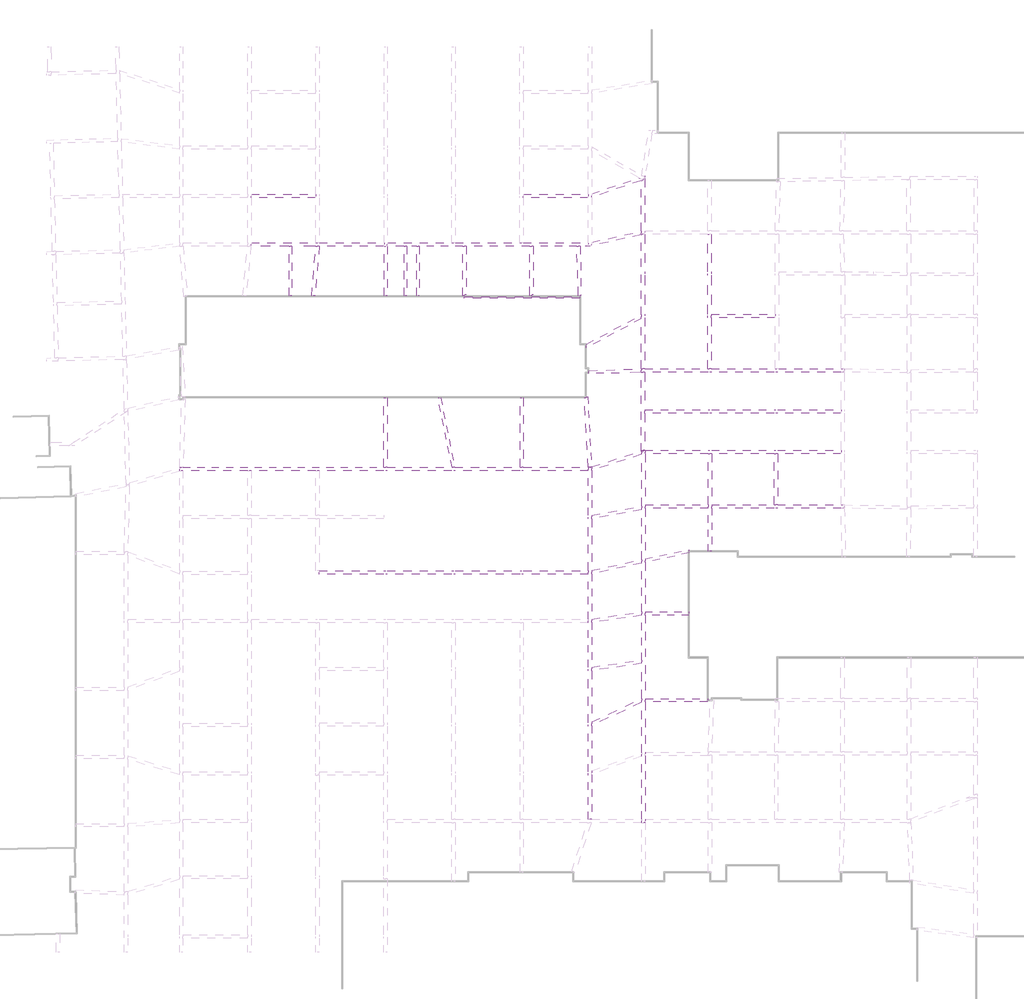
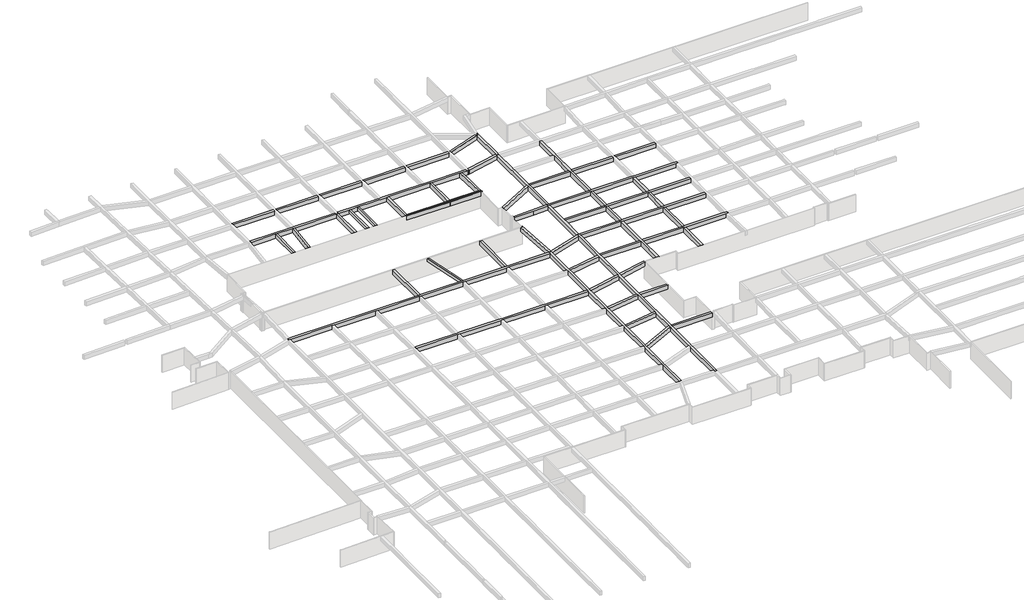
# One storey, part 12 of 20: 47 beams.
"""IFC4 building model written with IfcOpenShell, lengths in millimetres."""

import ifcopenshell
import ifcopenshell.guid

model = None  # the IFC model being written
_history = None  # IfcOwnerHistory: only IFC2X3 demands one
_inside = {}  # id of a spatial element -> (the spatial element, [elements in it])
_under = {}  # id of a project, library or spatial element -> (it, [spatial elements below it])
_declared = {}  # id of a project -> (the project, [libraries it declares])
_typed = {}  # id of a type object -> (the type object, [elements of that type])
_made_of = {}  # id of a material, layer set ... -> (it, [elements and type objects made of it])


def new_model(schema):
    """Start an empty IFC model of exactly this schema.

    Asked for "IFC4X3", IfcOpenShell would pick the latest addendum, in which some entities
    have other attributes; the version numbers below select the first issue.
    IFC2X3 requires an IfcOwnerHistory on every rooted entity: one is made here for all.
    """
    global model, _history
    if schema == "IFC4X3":
        model = ifcopenshell.file(schema_version=(4, 3, 0, 0))
    else:
        model = ifcopenshell.file(schema=schema)
    _inside.clear()
    _under.clear()
    _declared.clear()
    _typed.clear()
    _made_of.clear()
    _history = None
    if model.schema == "IFC2X3":
        org = make("IfcOrganization", Name="unknown")
        user = make(
            "IfcPersonAndOrganization",
            ThePerson=make("IfcPerson", FamilyName="unknown"),
            TheOrganization=org,
        )
        app = make(
            "IfcApplication",
            ApplicationDeveloper=org,
            Version="unknown",
            ApplicationFullName="unknown",
            ApplicationIdentifier="unknown",
        )
        _history = make(
            "IfcOwnerHistory",
            OwningUser=user,
            OwningApplication=app,
            ChangeAction="ADDED",
            CreationDate=0,
        )
    return model


def make(cls, **values):
    """One entity of the class cls with the attributes given. An attribute that is None is left unset."""
    return model.create_entity(
        cls, **{name: value for name, value in values.items() if value is not None}
    )


def rooted(cls, **values):
    """An entity with a GlobalId (a new one), such as an element, a storey or a relation."""
    return make(cls, GlobalId=ifcopenshell.guid.new(), OwnerHistory=_history, **values)


def si_unit(unit_type, name, prefix=None):
    """IfcSIUnit, for example si_unit("LENGTHUNIT", "METRE", prefix="MILLI")."""
    return make("IfcSIUnit", UnitType=unit_type, Prefix=prefix, Name=name)


def assignment(units):
    """IfcUnitAssignment: the units of a project."""
    return None if units is None else make("IfcUnitAssignment", Units=units)


def point(xyz):
    """IfcCartesianPoint."""
    return None if xyz is None else make("IfcCartesianPoint", Coordinates=xyz)


def direction(xyz):
    """IfcDirection."""
    return None if xyz is None else make("IfcDirection", DirectionRatios=xyz)


def frame(location, z_axis=None, x_axis=None):
    """IfcAxis2Placement3D, a coordinate frame: its origin and axes. An axis left out is left unset."""
    return make(
        "IfcAxis2Placement3D",
        Location=point(location),
        Axis=direction(z_axis),
        RefDirection=direction(x_axis),
    )


def origin():
    """The frame at (0, 0, 0) with its axes left unset."""
    return frame((0.0, 0.0, 0.0))


def place(relative_to, where):
    """IfcLocalPlacement: puts the frame where relative to a parent placement (None: the world)."""
    return make(
        "IfcLocalPlacement", PlacementRelTo=relative_to, RelativePlacement=where
    )


def context(
    kind, dimensions, precision=None, world=None, true_north=None, identifier=None
):
    """IfcGeometricRepresentationContext, for example the 3D "Model" context."""
    return make(
        "IfcGeometricRepresentationContext",
        ContextIdentifier=identifier,
        ContextType=kind,
        CoordinateSpaceDimension=dimensions,
        Precision=precision,
        WorldCoordinateSystem=world,
        TrueNorth=true_north,
    )


def project(units=None, contexts=None):
    """IfcProject with its units and contexts."""
    return rooted(
        "IfcProject",
        Name="project",
        RepresentationContexts=contexts,
        UnitsInContext=assignment(units),
    )


def spatial(cls, under=None, at=None, **own):
    """A site, building, storey or space (cls), placed at a placement, below another one or the project."""
    s = rooted(cls, ObjectPlacement=at, **own)
    if under is not None:
        _under.setdefault(under.id(), (under, []))[1].append(s)
    return s


def polyline(points):
    """IfcPolyline through the points."""
    return make("IfcPolyline", Points=[point(p) for p in points])


def outline(outer, holes=None, kind="AREA"):
    """IfcArbitraryClosedProfileDef: a profile drawn as a closed curve; with holes, ...WithVoids."""
    if holes is None:
        return make("IfcArbitraryClosedProfileDef", ProfileType=kind, OuterCurve=outer)
    return make(
        "IfcArbitraryProfileDefWithVoids",
        ProfileType=kind,
        OuterCurve=outer,
        InnerCurves=holes,
    )


def extrude(swept, where, along, depth):
    """IfcExtrudedAreaSolid: the profile swept, set in the frame where, extruded along a direction by depth."""
    return make(
        "IfcExtrudedAreaSolid",
        SweptArea=swept,
        Position=where,
        ExtrudedDirection=direction(along),
        Depth=depth,
    )


def faces_of(points, faces, orient=None, outer=None):
    """IfcFace entities. A face is a list of loops; a loop is a list of indices into points, from 0.

    orient and outer hold one flag for each loop. By default every Orientation is true, the
    first loop of a face is its IfcFaceOuterBound and the others are IfcFaceBound.
    """
    made = []
    for i, loops in enumerate(faces):
        bounds = []
        for j, loop in enumerate(loops):
            is_outer = j == 0 if outer is None else outer[i][j]
            bounds.append(
                make(
                    "IfcFaceOuterBound" if is_outer else "IfcFaceBound",
                    Bound=make("IfcPolyLoop", Polygon=[points[k] for k in loop]),
                    Orientation=True if orient is None else orient[i][j],
                )
            )
        made.append(make("IfcFace", Bounds=bounds))
    return made


def faceted_brep(points, faces, orient=None, outer=None, voids=None):
    """IfcFacetedBrep: a solid bounded by flat faces; with voids (closed shells), ...WithVoids."""
    shared = [point(p) for p in points]
    hull = make("IfcClosedShell", CfsFaces=faces_of(shared, faces, orient, outer))
    if voids is None:
        return make("IfcFacetedBrep", Outer=hull)
    return make(
        "IfcFacetedBrepWithVoids",
        Outer=hull,
        Voids=[
            make(cls, CfsFaces=faces_of(shared, fs, o, b)) for cls, fs, o, b in voids
        ],
    )


def shape(context_of_items, identifier, shape_type, items):
    """IfcShapeRepresentation: the items that make up one representation, for example the "Body"."""
    return make(
        "IfcShapeRepresentation",
        ContextOfItems=context_of_items,
        RepresentationIdentifier=identifier,
        RepresentationType=shape_type,
        Items=items,
    )


def made_of(thing, what):
    """Note that an element or type object is made of a material, layer set ...; save() writes the relation."""
    if what is not None:
        _made_of.setdefault(what.id(), (what, []))[1].append(thing)
    return thing


def element(
    cls,
    number,
    at=None,
    inside=None,
    cuts=None,
    type_object=None,
    material=None,
    context=None,
    identifier="Body",
    shape_type=None,
    held_by="IfcProductDefinitionShape",
    body=None,
    shapes=None,
    **own,
):
    """One element of the class cls, such as IfcWall. Its Tag is "e" and its number.

    at: its placement. inside: the storey or other place that contains it. cuts: it is an
    opening in that element (IfcRelVoidsElement). A single representation is given by context,
    identifier, shape_type and body (its items); several are given by shapes. held_by: the class
    of the entity that holds the representations. save() writes the other relations.
    """
    e = rooted(cls, Tag="e%d" % number, ObjectPlacement=at, **own)
    if body is not None:
        shapes = [shape(context, identifier, shape_type, body)]
    if shapes is not None:
        e.Representation = make(held_by, Representations=shapes)
    if inside is not None:
        _inside.setdefault(inside.id(), (inside, []))[1].append(e)
    if cuts is not None:
        rooted(
            "IfcRelVoidsElement", RelatingBuildingElement=cuts, RelatedOpeningElement=e
        )
    if type_object is not None:
        _typed.setdefault(type_object.id(), (type_object, []))[1].append(e)
    return made_of(e, material)


def aggregate(whole, parts):
    """IfcRelAggregates: a whole, such as a stair, and the parts it consists of."""
    return rooted("IfcRelAggregates", RelatingObject=whole, RelatedObjects=parts)


def save(model, path):
    """Write the relations noted so far, then the file.

    IfcRelAggregates (storeys below a building ...), IfcRelContainedInSpatialStructure (elements
    in a storey), IfcRelDefinesByType, IfcRelAssociatesMaterial and IfcRelDeclares: one each for
    every whole, place, type object, material and project.
    """
    for whole, parts in _under.values():
        aggregate(whole, parts)
    for where, things in _inside.values():
        rooted(
            "IfcRelContainedInSpatialStructure",
            RelatedElements=things,
            RelatingStructure=where,
        )
    for kind, things in _typed.values():
        rooted("IfcRelDefinesByType", RelatedObjects=things, RelatingType=kind)
    for what, things in _made_of.values():
        rooted("IfcRelAssociatesMaterial", RelatedObjects=things, RelatingMaterial=what)
    for by, libraries in _declared.values():
        rooted("IfcRelDeclares", RelatingContext=by, RelatedDefinitions=libraries)
    model.write(path)


model = new_model("IFC4")

# Units and contexts
model_context = context("Model", 3, world=origin())
ifc_project = project(units=[si_unit("LENGTHUNIT", "METRE", prefix="MILLI")], contexts=[model_context])

# Site, building, storey
site = spatial("IfcSite", under=ifc_project)
building = spatial("IfcBuilding", under=site)
storey = spatial("IfcBuildingStorey", under=building, Name="户型图", Elevation=0.0)

# Beams
placement = place(None, origin())
element("IfcBeam", 1, ObjectType="混凝土 - 矩形梁 : KL_beam", at=placement, inside=storey, context=model_context, shape_type="SweptSolid", body=[
    extrude(outline(polyline([(62850.0, 125365.1975441), (62850.0, 125765.1975441), (70471.1713568, 125765.1975441), (70471.1713568, 125365.1975441), (62850.0, 125365.1975441)])), frame((0.0, 0.0, 2500.0), z_axis=(0.0, 0.0, 1.0), x_axis=(1.0, 0.0, 0.0)), (0.0, 0.0, 1.0), 800.0),
    extrude(outline(polyline([(78471.1713568, 125765.1975441), (78471.1713568, 125365.1975441), (70871.1713568, 125365.1975441), (70871.1713568, 125765.1975441), (78471.1713568, 125765.1975441)])), frame((0.0, 0.0, 2500.0), z_axis=(0.0, 0.0, 1.0), x_axis=(1.0, 0.0, 0.0)), (0.0, 0.0, 1.0), 800.0),
])
element("IfcBeam", 2, ObjectType="混凝土 - 矩形梁 : KL_beam", at=placement, inside=storey, context=model_context, shape_type="Brep", body=[
    faceted_brep([(78471.1713568, 119690.0, 3300.0), (78471.1713568, 120090.0, 3300.0), (70871.1713568, 120090.0, 3300.0), (70471.1713568, 120090.0, 3300.0), (62850.0, 120090.0, 3300.0), (62850.0, 119690.0, 3300.0), (67321.1713568, 119690.0, 3300.0), (67621.1713568, 119690.0, 3300.0), (70454.1162605, 119690.0, 3300.0), (70855.4563641, 119690.0, 3300.0), (78471.1713568, 119690.0, 2500.0), (62850.0, 119690.0, 2500.0), (70454.1162605, 119690.0, 2500.0), (70855.4563641, 119690.0, 2500.0), (78471.1713568, 120090.0, 2500.0), (62850.0, 120090.0, 2500.0), (70471.1713568, 120090.0, 2500.0), (70871.1713568, 120090.0, 2500.0)], [[[0, 1, 2, 3, 4, 5, 6, 7, 8, 9]], [[10, 0, 9, 8, 7, 6, 5, 11, 12, 13]], [[14, 10, 13, 12, 11, 15, 16, 17]], [[1, 14, 17, 16, 15, 4, 3, 2]], [[1, 0, 10, 14]], [[5, 4, 15, 11]]]),
])
element("IfcBeam", 3, ObjectType="混凝土 - 矩形梁 : KL_beam", at=placement, inside=storey, context=model_context, shape_type="SweptSolid", body=[
    extrude(outline(polyline([(78871.1713568, 125365.1975441), (78871.1713568, 125765.1975441), (86450.0, 125765.1975441), (86450.0, 125365.1975441), (78871.1713568, 125365.1975441)])), frame((0.0, 0.0, 2500.0), z_axis=(0.0, 0.0, 1.0), x_axis=(1.0, 0.0, 0.0)), (0.0, 0.0, 1.0), 800.0),
    extrude(outline(polyline([(102450.0, 125765.1975441), (102450.0, 125365.1975441), (94823.4648002, 125365.1975441), (94823.4648002, 125765.1975441), (102450.0, 125765.1975441)])), frame((0.0, 0.0, 2500.0), z_axis=(0.0, 0.0, 1.0), x_axis=(1.0, 0.0, 0.0)), (0.0, 0.0, 1.0), 800.0),
    extrude(outline(polyline([(94423.4648002, 125765.1975441), (94423.4648002, 125365.1975441), (86850.0, 125365.1975441), (86850.0, 125765.1975441), (94423.4648002, 125765.1975441)])), frame((0.0, 0.0, 2500.0), z_axis=(0.0, 0.0, 1.0), x_axis=(1.0, 0.0, 0.0)), (0.0, 0.0, 1.0), 800.0),
])
element("IfcBeam", 4, ObjectType="混凝土 - 矩形梁 : KL_beam", at=placement, inside=storey, context=model_context, shape_type="Brep", body=[
    faceted_brep([(108863.5483185, 127442.6599197, 3300.0), (108401.581434, 127709.3766248, 3300.0), (102850.0, 125843.4152433, 3300.0), (102850.0, 125421.4252388, 3300.0), (108685.3829072, 127382.7761225, 3300.0), (108863.5483185, 127442.6599197, 2500.0), (102850.0, 125421.4252388, 2500.0), (108685.3829072, 127382.7761225, 2500.0), (108401.581434, 127709.3766248, 2500.0), (102850.0, 125843.4152433, 2500.0)], [[[0, 1, 2, 3, 4]], [[5, 0, 4, 3, 6, 7]], [[8, 5, 7, 6, 9]], [[1, 8, 9, 2]], [[1, 0, 5, 8]], [[3, 2, 9, 6]]]),
])
element("IfcBeam", 5, ObjectType="混凝土 - 矩形梁 : KL_beam", at=placement, inside=storey, context=model_context, shape_type="Brep", body=[
    faceted_brep([(108907.217496, 127879.3277237, 3300.0), (109063.5483185, 127789.0700812, 3300.0), (108863.5483185, 127442.6599197, 3300.0), (108685.3829072, 127382.7761225, 3300.0), (108685.3829072, 121449.0992016, 3300.0), (108685.3829072, 121039.1549065, 3300.0), (108907.5439108, 121089.0, 3300.0), (109085.3829072, 121128.9007984, 3300.0), (109085.3829072, 121489.0, 3300.0), (109085.3829072, 127645.2534803, 3300.0), (109085.3829072, 127939.2115209, 3300.0), (108685.3829072, 121039.1549065, 2500.0), (108685.3829072, 127382.7761225, 2500.0), (108685.3829072, 121449.0992016, 2500.0), (109063.5483185, 127789.0700812, 2500.0), (108907.217496, 127879.3277237, 2500.0), (109085.3829072, 127939.2115209, 2500.0), (109085.3829072, 127645.2534803, 2500.0), (109085.3829072, 121489.0, 2500.0), (109085.3829072, 121128.9007984, 2500.0), (108907.5439108, 121089.0, 2500.0), (108863.5483185, 127442.6599197, 2500.0)], [[[0, 1, 2, 3, 4, 5, 6, 7, 8, 9, 10]], [[11, 5, 4, 3, 12, 13]], [[14, 15, 16, 17, 18, 19, 20, 11, 13, 12, 21]], [[7, 19, 18, 17, 16, 10, 9, 8]], [[15, 0, 10, 16]], [[1, 0, 15, 14]], [[3, 2, 21, 12]], [[7, 6, 5, 11, 20, 19]], [[1, 14, 21, 2]]]),
])
element("IfcBeam", 6, ObjectType="混凝土 - 矩形梁 : KL_beam", at=placement, inside=storey, context=model_context, shape_type="SweptSolid", body=[
    extrude(outline(polyline([(102850.0, 119729.9007984), (102850.0, 120139.8450935), (108685.3829072, 121449.0992016), (108685.3829072, 121039.1549065), (102850.0, 119729.9007984)])), frame((0.0, 0.0, 2500.0), z_axis=(0.0, 0.0, 1.0), x_axis=(1.0, 0.0, 0.0)), (0.0, 0.0, 1.0), 800.0),
])
element("IfcBeam", 7, ObjectType="混凝土 - 矩形梁 : KL_beam", at=placement, inside=storey, context=model_context, shape_type="Brep", body=[
    faceted_brep([(102672.1610035, 119690.0, 3300.0), (102850.0, 119729.9007984, 3300.0), (102450.0, 119729.9007984, 3300.0), (102450.0, 120050.0992016, 3300.0), (102450.0, 120090.0, 3300.0), (94823.4648002, 120090.0, 3300.0), (94423.4648002, 120090.0, 3300.0), (86850.0, 120090.0, 3300.0), (86450.0, 120090.0, 3300.0), (78871.1713568, 120090.0, 3300.0), (78871.1713568, 119690.0, 3300.0), (80821.1713568, 119690.0, 3300.0), (81121.1713568, 119690.0, 3300.0), (82321.1713568, 119690.0, 3300.0), (82621.1713568, 119690.0, 3300.0), (87704.0, 119690.0, 3300.0), (88104.0, 119690.0, 3300.0), (95604.0, 119690.0, 3300.0), (96004.0, 119690.0, 3300.0), (101098.0899965, 119690.0, 3300.0), (101498.3338142, 119690.0, 3300.0), (102672.1610035, 119690.0, 2500.0), (78871.1713568, 119690.0, 2500.0), (87704.0, 119690.0, 2500.0), (88104.0, 119690.0, 2500.0), (95604.0, 119690.0, 2500.0), (96004.0, 119690.0, 2500.0), (101098.0899965, 119690.0, 2500.0), (101498.3338142, 119690.0, 2500.0), (102850.0, 119729.9007984, 2500.0), (78871.1713568, 120090.0, 2500.0), (86450.0, 120090.0, 2500.0), (86850.0, 120090.0, 2500.0), (94423.4648002, 120090.0, 2500.0), (94823.4648002, 120090.0, 2500.0), (102450.0, 120090.0, 2500.0), (102450.0, 120050.0992016, 2500.0), (102450.0, 119729.9007984, 2500.0)], [[[0, 1, 2, 3, 4, 5, 6, 7, 8, 9, 10, 11, 12, 13, 14, 15, 16, 17, 18, 19, 20]], [[21, 0, 20, 19, 18, 17, 16, 15, 14, 13, 12, 11, 10, 22, 23, 24, 25, 26, 27, 28]], [[29, 21, 28, 27, 26, 25, 24, 23, 22, 30, 31, 32, 33, 34, 35, 36, 37]], [[4, 35, 34, 33, 32, 31, 30, 9, 8, 7, 6, 5]], [[1, 0, 21, 29]], [[2, 37, 36, 35, 4, 3]], [[37, 2, 1, 29]], [[10, 9, 30, 22]]]),
])
element("IfcBeam", 8, ObjectType="混凝土 - 矩形梁 : KL_beam", at=placement, inside=storey, context=model_context, shape_type="Brep", body=[
    faceted_brep([(70850.0, 81560.0, 3300.0), (70850.0, 81160.0, 3300.0), (78450.0, 81160.0, 3300.0), (78850.0, 81160.0, 3300.0), (86450.0, 81160.0, 3300.0), (86850.0, 81160.0, 3300.0), (94450.0, 81160.0, 3300.0), (94850.0, 81160.0, 3300.0), (102445.0, 81160.0, 3300.0), (102445.0, 81560.0, 3300.0), (94850.0, 81560.0, 3300.0), (94450.0, 81560.0, 3300.0), (86850.0, 81560.0, 3300.0), (86450.0, 81560.0, 3300.0), (78850.0, 81560.0, 3300.0), (78450.0, 81560.0, 3300.0), (70850.0, 81160.0, 2500.0), (78450.0, 81160.0, 2500.0), (78850.0, 81160.0, 2500.0), (86450.0, 81160.0, 2500.0), (86850.0, 81160.0, 2500.0), (94450.0, 81160.0, 2500.0), (94850.0, 81160.0, 2500.0), (102445.0, 81160.0, 2500.0), (70850.0, 81560.0, 2500.0), (78450.0, 81560.0, 2500.0), (78850.0, 81560.0, 2500.0), (86450.0, 81560.0, 2500.0), (86850.0, 81560.0, 2500.0), (94450.0, 81560.0, 2500.0), (94850.0, 81560.0, 2500.0), (102445.0, 81560.0, 2500.0)], [[[0, 1, 2, 3, 4, 5, 6, 7, 8, 9, 10, 11, 12, 13, 14, 15]], [[1, 16, 17, 18, 19, 20, 21, 22, 23, 8, 7, 6, 5, 4, 3, 2]], [[16, 24, 25, 26, 27, 28, 29, 30, 31, 23, 22, 21, 20, 19, 18, 17]], [[24, 0, 15, 14, 13, 12, 11, 10, 9, 31, 30, 29, 28, 27, 26, 25]], [[1, 0, 24, 16]], [[9, 8, 23, 31]]]),
])
element("IfcBeam", 9, ObjectType="混凝土 - 矩形梁 : KL_beam", at=placement, inside=storey, context=model_context, shape_type="Brep", body=[
    faceted_brep([(102845.0, 93710.0, 3300.0), (102614.3346246, 93710.0, 3300.0), (102445.0, 93710.0, 3300.0), (102445.0, 93310.0, 3300.0), (102445.0, 88060.0, 3300.0), (102445.0, 87660.0, 3300.0), (102445.0, 81560.0, 3300.0), (102445.0, 81160.0, 3300.0), (102445.0, 75860.0, 3300.0), (102445.0, 75460.0, 3300.0), (102445.0, 70210.0, 3300.0), (102445.0, 69810.0, 3300.0), (102445.0, 63683.0, 3300.0), (102445.0, 63283.0, 3300.0), (102445.0, 57960.0, 3300.0), (102445.0, 57560.0, 3300.0), (102445.0, 52365.0, 3300.0), (102845.0, 52365.0, 3300.0), (102845.0, 57619.9584924, 3300.0), (102845.0, 58045.6296013, 3300.0), (102845.0, 63355.5859478, 3300.0), (102845.0, 63796.9371154, 3300.0), (102845.0, 69836.1426524, 3300.0), (102845.0, 70240.0736814, 3300.0), (102845.0, 75486.1426524, 3300.0), (102845.0, 75890.0736814, 3300.0), (102845.0, 81198.0431934, 3300.0), (102845.0, 81606.9794313, 3300.0), (102845.0, 87692.1800738, 3300.0), (102845.0, 88098.3507185, 3300.0), (102845.0, 93363.1772493, 3300.0), (102445.0, 93710.0, 2500.0), (102445.0, 93310.0, 2500.0), (102445.0, 88060.0, 2500.0), (102445.0, 87660.0, 2500.0), (102445.0, 81560.0, 2500.0), (102445.0, 81160.0, 2500.0), (102445.0, 75860.0, 2500.0), (102445.0, 75460.0, 2500.0), (102445.0, 70210.0, 2500.0), (102445.0, 69810.0, 2500.0), (102445.0, 63683.0, 2500.0), (102445.0, 63283.0, 2500.0), (102445.0, 57960.0, 2500.0), (102445.0, 57560.0, 2500.0), (102445.0, 52365.0, 2500.0), (102614.3346246, 93710.0, 2500.0), (102845.0, 93710.0, 2500.0), (102845.0, 93363.1772493, 2500.0), (102845.0, 88098.3507185, 2500.0), (102845.0, 87692.1800738, 2500.0), (102845.0, 81606.9794313, 2500.0), (102845.0, 81198.0431934, 2500.0), (102845.0, 75890.0736814, 2500.0), (102845.0, 75486.1426524, 2500.0), (102845.0, 70240.0736814, 2500.0), (102845.0, 69836.1426524, 2500.0), (102845.0, 63796.9371154, 2500.0), (102845.0, 63355.5859478, 2500.0), (102845.0, 58045.6296013, 2500.0), (102845.0, 57619.9584924, 2500.0), (102845.0, 52365.0, 2500.0)], [[[0, 1, 2, 3, 4, 5, 6, 7, 8, 9, 10, 11, 12, 13, 14, 15, 16, 17, 18, 19, 20, 21, 22, 23, 24, 25, 26, 27, 28, 29, 30]], [[2, 31, 32, 33, 34, 35, 36, 37, 38, 39, 40, 41, 42, 43, 44, 45, 16, 15, 14, 13, 12, 11, 10, 9, 8, 7, 6, 5, 4, 3]], [[31, 46, 47, 48, 49, 50, 51, 52, 53, 54, 55, 56, 57, 58, 59, 60, 61, 45, 44, 43, 42, 41, 40, 39, 38, 37, 36, 35, 34, 33, 32]], [[47, 0, 30, 29, 28, 27, 26, 25, 24, 23, 22, 21, 20, 19, 18, 17, 61, 60, 59, 58, 57, 56, 55, 54, 53, 52, 51, 50, 49, 48]], [[2, 1, 0, 47, 46, 31]], [[17, 16, 45, 61]]]),
])
element("IfcBeam", 10, ObjectType="混凝土 - 矩形梁 : KL_beam", at=placement, inside=storey, context=model_context, shape_type="Brep", body=[
    faceted_brep([(109150.0, 95636.8227507, 3300.0), (108750.0, 95636.8227507, 3300.0), (108750.0, 95217.5626577, 3300.0), (108750.0, 89139.5615396, 3300.0), (108750.0, 88733.3908948, 3300.0), (108750.0, 82862.125928, 3300.0), (108750.0, 82453.18969, 3300.0), (108750.0, 76719.9673104, 3300.0), (108750.0, 76316.0362814, 3300.0), (108750.0, 71069.9673104, 3300.0), (108750.0, 70666.0362814, 3300.0), (108750.0, 66550.4838368, 3300.0), (108750.0, 66109.1326692, 3300.0), (108750.0, 60194.8738347, 3300.0), (108750.0, 59769.2027257, 3300.0), (108750.0, 52365.0, 3300.0), (108750.0, 51965.0, 3300.0), (109150.0, 51965.0, 3300.0), (109150.0, 52365.0, 3300.0), (109150.0, 59854.832327, 3300.0), (109150.0, 60254.832327, 3300.0), (109150.0, 66143.0, 3300.0), (109150.0, 66543.0, 3300.0), (109150.0, 76346.1099628, 3300.0), (109150.0, 76746.1099628, 3300.0), (109150.0, 82538.8952678, 3300.0), (109150.0, 82948.1944468, 3300.0), (109150.0, 88890.0, 3300.0), (109150.0, 89290.0, 3300.0), (109150.0, 95290.0, 3300.0), (108750.0, 95636.8227507, 2500.0), (108750.0, 95217.5626577, 2500.0), (108750.0, 89139.5615396, 2500.0), (108750.0, 88733.3908948, 2500.0), (108750.0, 82862.125928, 2500.0), (108750.0, 82453.18969, 2500.0), (108750.0, 76719.9673104, 2500.0), (108750.0, 76316.0362814, 2500.0), (108750.0, 71069.9673104, 2500.0), (108750.0, 70666.0362814, 2500.0), (108750.0, 66550.4838368, 2500.0), (108750.0, 66109.1326692, 2500.0), (108750.0, 60194.8738347, 2500.0), (108750.0, 59769.2027257, 2500.0), (108750.0, 52365.0, 2500.0), (108750.0, 51965.0, 2500.0), (109150.0, 95636.8227507, 2500.0), (109150.0, 95290.0, 2500.0), (109150.0, 89290.0, 2500.0), (109150.0, 88890.0, 2500.0), (109150.0, 82948.1944468, 2500.0), (109150.0, 82538.8952678, 2500.0), (109150.0, 76746.1099628, 2500.0), (109150.0, 76346.1099628, 2500.0), (109150.0, 66543.0, 2500.0), (109150.0, 66143.0, 2500.0), (109150.0, 60254.832327, 2500.0), (109150.0, 59854.832327, 2500.0), (109150.0, 52365.0, 2500.0), (109150.0, 51965.0, 2500.0)], [[[0, 1, 2, 3, 4, 5, 6, 7, 8, 9, 10, 11, 12, 13, 14, 15, 16, 17, 18, 19, 20, 21, 22, 23, 24, 25, 26, 27, 28, 29]], [[1, 30, 31, 32, 33, 34, 35, 36, 37, 38, 39, 40, 41, 42, 43, 44, 45, 16, 15, 14, 13, 12, 11, 10, 9, 8, 7, 6, 5, 4, 3, 2]], [[30, 46, 47, 48, 49, 50, 51, 52, 53, 54, 55, 56, 57, 58, 59, 45, 44, 43, 42, 41, 40, 39, 38, 37, 36, 35, 34, 33, 32, 31]], [[46, 0, 29, 28, 27, 26, 25, 24, 23, 22, 21, 20, 19, 18, 17, 59, 58, 57, 56, 55, 54, 53, 52, 51, 50, 49, 48, 47]], [[0, 46, 30, 1]], [[17, 16, 45, 59]]]),
])
element("IfcBeam", 11, ObjectType="混凝土 - 矩形梁 : KL_beam", at=placement, inside=storey, context=model_context, shape_type="Brep", body=[
    faceted_brep([(54450.0, 93710.0, 3300.0), (54450.0, 93659.5803713, 3300.0), (54450.0, 93310.0, 3300.0), (54850.0, 93310.0, 3300.0), (62450.0, 93310.0, 3300.0), (62850.0, 93310.0, 3300.0), (70450.0, 93310.0, 3300.0), (70850.0, 93310.0, 3300.0), (78450.0, 93310.0, 3300.0), (78850.0, 93310.0, 3300.0), (86450.0, 93310.0, 3300.0), (86850.0, 93310.0, 3300.0), (94450.0, 93310.0, 3300.0), (94850.0, 93310.0, 3300.0), (102445.0, 93310.0, 3300.0), (102445.0, 93710.0, 3300.0), (102433.8972182, 93710.0, 3300.0), (94850.0, 93710.0, 3300.0), (94450.0, 93710.0, 3300.0), (86762.8978362, 93710.0, 3300.0), (86456.9315437, 93710.0, 3300.0), (78850.0, 93710.0, 3300.0), (78450.0, 93710.0, 3300.0), (54856.0147831, 93710.0, 3300.0), (54621.1541992, 93710.0, 3300.0), (54455.8391762, 93710.0, 3300.0), (54450.0, 93310.0, 2500.0), (54850.0, 93310.0, 2500.0), (62450.0, 93310.0, 2500.0), (62850.0, 93310.0, 2500.0), (70450.0, 93310.0, 2500.0), (70850.0, 93310.0, 2500.0), (78450.0, 93310.0, 2500.0), (78850.0, 93310.0, 2500.0), (86450.0, 93310.0, 2500.0), (86850.0, 93310.0, 2500.0), (94450.0, 93310.0, 2500.0), (94850.0, 93310.0, 2500.0), (102445.0, 93310.0, 2500.0), (54450.0, 93659.5803713, 2500.0), (54450.0, 93710.0, 2500.0), (54455.8391762, 93710.0, 2500.0), (54621.1541992, 93710.0, 2500.0), (54856.0147831, 93710.0, 2500.0), (78450.0, 93710.0, 2500.0), (78850.0, 93710.0, 2500.0), (94450.0, 93710.0, 2500.0), (94850.0, 93710.0, 2500.0), (102433.8972182, 93710.0, 2500.0), (102445.0, 93710.0, 2500.0)], [[[0, 1, 2, 3, 4, 5, 6, 7, 8, 9, 10, 11, 12, 13, 14, 15, 16, 17, 18, 19, 20, 21, 22, 23, 24, 25]], [[2, 26, 27, 28, 29, 30, 31, 32, 33, 34, 35, 36, 37, 38, 14, 13, 12, 11, 10, 9, 8, 7, 6, 5, 4, 3]], [[26, 39, 40, 41, 42, 43, 44, 45, 46, 47, 48, 49, 38, 37, 36, 35, 34, 33, 32, 31, 30, 29, 28, 27]], [[40, 0, 25, 24, 23, 22, 21, 20, 19, 18, 17, 16, 15, 49, 48, 47, 46, 45, 44, 43, 42, 41]], [[15, 14, 38, 49]], [[2, 1, 0, 40, 39, 26]]]),
])
element("IfcBeam", 12, ObjectType="混凝土 - 矩形梁 : KL_beam", at=placement, inside=storey, context=model_context, shape_type="Brep", body=[
    faceted_brep([(102845.0, 93710.0, 3300.0), (102845.0, 93363.1772493, 3300.0), (108750.0, 95217.5626577, 3300.0), (108750.0, 95636.8227507, 3300.0), (108747.6070916, 95636.0712902, 3300.0), (108685.3829072, 95616.5306264, 3300.0), (102830.806561, 93777.9800847, 3300.0), (102614.3346246, 93710.0, 3300.0), (102845.0, 93363.1772493, 2500.0), (108750.0, 95217.5626577, 2500.0), (102845.0, 93710.0, 2500.0), (102614.3346246, 93710.0, 2500.0), (102830.806561, 93777.9800847, 2500.0), (108685.3829072, 95616.5306264, 2500.0), (108747.6070916, 95636.0712902, 2500.0), (108750.0, 95636.8227507, 2500.0)], [[[0, 1, 2, 3, 4, 5, 6, 7]], [[1, 8, 9, 2]], [[8, 10, 11, 12, 13, 14, 15, 9]], [[11, 7, 6, 5, 4, 3, 15, 14, 13, 12]], [[0, 10, 8, 1]], [[10, 0, 7, 11]], [[3, 2, 9, 15]]]),
])
element("IfcBeam", 13, ObjectType="混凝土 - 矩形梁 : KL_beam", at=placement, inside=storey, context=model_context, shape_type="SweptSolid", body=[
    extrude(outline(polyline([(102845.0, 87692.1800738), (102845.0, 88098.3507185), (108750.0, 89139.5615396), (108750.0, 88733.3908948), (102845.0, 87692.1800738)])), frame((0.0, 0.0, 2500.0), z_axis=(0.0, 0.0, 1.0), x_axis=(1.0, 0.0, 0.0)), (0.0, 0.0, 1.0), 800.0),
])
element("IfcBeam", 14, ObjectType="混凝土 - 矩形梁 : KL_beam", at=placement, inside=storey, context=model_context, shape_type="SweptSolid", body=[
    extrude(outline(polyline([(102845.0, 81198.0431934), (102845.0, 81606.9794313), (108750.0, 82862.125928), (108750.0, 82453.18969), (102845.0, 81198.0431934)])), frame((0.0, 0.0, 2500.0), z_axis=(0.0, 0.0, 1.0), x_axis=(1.0, 0.0, 0.0)), (0.0, 0.0, 1.0), 800.0),
])
element("IfcBeam", 15, ObjectType="混凝土 - 矩形梁 : KL_beam", at=placement, inside=storey, context=model_context, shape_type="SweptSolid", body=[
    extrude(outline(polyline([(102845.0, 75486.1426524), (102845.0, 75890.0736814), (108750.0, 76719.9673104), (108750.0, 76316.0362814), (102845.0, 75486.1426524)])), frame((0.0, 0.0, 2500.0), z_axis=(0.0, 0.0, 1.0), x_axis=(1.0, 0.0, 0.0)), (0.0, 0.0, 1.0), 800.0),
])
element("IfcBeam", 16, ObjectType="混凝土 - 矩形梁 : KL_beam", at=placement, inside=storey, context=model_context, shape_type="SweptSolid", body=[
    extrude(outline(polyline([(102845.0, 69836.1426524), (102845.0, 70240.0736814), (108750.0, 71069.9673104), (108750.0, 70666.0362814), (102845.0, 69836.1426524)])), frame((0.0, 0.0, 2500.0), z_axis=(0.0, 0.0, 1.0), x_axis=(1.0, 0.0, 0.0)), (0.0, 0.0, 1.0), 800.0),
])
element("IfcBeam", 17, ObjectType="混凝土 - 矩形梁 : KL_beam", at=placement, inside=storey, context=model_context, shape_type="SweptSolid", body=[
    extrude(outline(polyline([(102845.0, 63355.5859478), (102845.0, 63796.9371154), (108750.0, 66550.4838368), (108750.0, 66109.1326692), (102845.0, 63355.5859478)])), frame((0.0, 0.0, 2500.0), z_axis=(0.0, 0.0, 1.0), x_axis=(1.0, 0.0, 0.0)), (0.0, 0.0, 1.0), 800.0),
])
element("IfcBeam", 18, ObjectType="混凝土 - 矩形梁 : KL_beam", at=placement, inside=storey, context=model_context, shape_type="SweptSolid", body=[
    extrude(outline(polyline([(116491.0, 66543.0), (116491.0, 66143.0), (109150.0, 66143.0), (109150.0, 66543.0), (116491.0, 66543.0)])), frame((0.0, 0.0, 2500.0), z_axis=(0.0, 0.0, 1.0), x_axis=(1.0, 0.0, 0.0)), (0.0, 0.0, 1.0), 800.0),
])
element("IfcBeam", 19, ObjectType="混凝土 - 矩形梁 : KL_beam", at=placement, inside=storey, context=model_context, shape_type="SweptSolid", body=[
    extrude(outline(polyline([(114284.0, 76746.1099628), (114284.0, 76346.1099628), (109150.0, 76346.1099628), (109150.0, 76746.1099628), (114284.0, 76746.1099628)])), frame((0.0, 0.0, 2500.0), z_axis=(0.0, 0.0, 1.0), x_axis=(1.0, 0.0, 0.0)), (0.0, 0.0, 1.0), 800.0),
])
element("IfcBeam", 20, ObjectType="混凝土 - 矩形梁 : KL_beam", at=placement, inside=storey, context=model_context, shape_type="SweptSolid", body=[
    extrude(outline(polyline([(114241.6075264, 84052.4555658), (114326.3880257, 83661.5434696), (109150.0, 82538.8952678), (109150.0, 82948.1944468), (114241.6075264, 84052.4555658)])), frame((0.0, 0.0, 2500.0), z_axis=(0.0, 0.0, 1.0), x_axis=(1.0, 0.0, 0.0)), (0.0, 0.0, 1.0), 800.0),
])
element("IfcBeam", 21, ObjectType="混凝土 - 矩形梁 : KL_beam", at=placement, inside=storey, context=model_context, shape_type="SweptSolid", body=[
    extrude(outline(polyline([(109150.0, 88890.0), (109150.0, 89290.0), (116544.0, 89290.0), (116544.0, 88890.0), (109150.0, 88890.0)])), frame((0.0, 0.0, 2500.0), z_axis=(0.0, 0.0, 1.0), x_axis=(1.0, 0.0, 0.0)), (0.0, 0.0, 1.0), 800.0),
])
element("IfcBeam", 22, ObjectType="混凝土 - 矩形梁 : KL_beam", at=placement, inside=storey, context=model_context, shape_type="Brep", body=[
    faceted_brep([(132555.1324416, 88890.0, 3300.0), (132550.0, 89092.5337107, 3300.0), (132544.9959727, 89290.0, 3300.0), (132150.0, 89290.0, 3300.0), (124697.0, 89290.0, 3300.0), (124297.0, 89290.0, 3300.0), (116944.0, 89290.0, 3300.0), (116944.0, 88890.0, 3300.0), (124297.0, 88890.0, 3300.0), (124697.0, 88890.0, 3300.0), (132155.0040273, 88890.0, 3300.0), (132555.1324416, 88890.0, 2500.0), (116944.0, 88890.0, 2500.0), (124297.0, 88890.0, 2500.0), (124697.0, 88890.0, 2500.0), (132155.0040273, 88890.0, 2500.0), (132544.9959727, 89290.0, 2500.0), (132550.0, 89092.5337107, 2500.0), (116944.0, 89290.0, 2500.0), (124297.0, 89290.0, 2500.0), (124697.0, 89290.0, 2500.0), (132150.0, 89290.0, 2500.0)], [[[0, 1, 2, 3, 4, 5, 6, 7, 8, 9, 10]], [[11, 0, 10, 9, 8, 7, 12, 13, 14, 15]], [[16, 17, 11, 15, 14, 13, 12, 18, 19, 20, 21]], [[2, 16, 21, 20, 19, 18, 6, 5, 4, 3]], [[7, 6, 18, 12]], [[2, 1, 0, 11, 17, 16]]]),
])
element("IfcBeam", 23, ObjectType="混凝土 - 矩形梁 : KL_beam", at=placement, inside=storey, context=model_context, shape_type="Brep", body=[
    faceted_brep([(108750.0, 95636.8227507, 3300.0), (109150.0, 95636.8227507, 3300.0), (109150.0, 95343.1772493, 3300.0), (109150.0, 95290.0, 3300.0), (116544.0, 95290.0, 3300.0), (116944.0, 95290.0, 3300.0), (124297.0, 95290.0, 3300.0), (124697.0, 95290.0, 3300.0), (132150.0, 95290.0, 3300.0), (132150.0, 95690.0, 3300.0), (124697.0, 95690.0, 3300.0), (124297.0, 95690.0, 3300.0), (116944.0, 95690.0, 3300.0), (116544.0, 95690.0, 3300.0), (109085.3829072, 95690.0, 3300.0), (108747.6070916, 95690.0, 3300.0), (108747.6070916, 95636.0712902, 3300.0), (109150.0, 95290.0, 2500.0), (116544.0, 95290.0, 2500.0), (116944.0, 95290.0, 2500.0), (124297.0, 95290.0, 2500.0), (124697.0, 95290.0, 2500.0), (132150.0, 95290.0, 2500.0), (109150.0, 95636.8227507, 2500.0), (108750.0, 95636.8227507, 2500.0), (108747.6070916, 95636.0712902, 2500.0), (108747.6070916, 95690.0, 2500.0), (109085.3829072, 95690.0, 2500.0), (116544.0, 95690.0, 2500.0), (116944.0, 95690.0, 2500.0), (124297.0, 95690.0, 2500.0), (124697.0, 95690.0, 2500.0), (132150.0, 95690.0, 2500.0), (109150.0, 95343.1772493, 2500.0)], [[[0, 1, 2, 3, 4, 5, 6, 7, 8, 9, 10, 11, 12, 13, 14, 15, 16]], [[3, 17, 18, 19, 20, 21, 22, 8, 7, 6, 5, 4]], [[23, 24, 25, 26, 27, 28, 29, 30, 31, 32, 22, 21, 20, 19, 18, 17, 33]], [[26, 15, 14, 13, 12, 11, 10, 9, 32, 31, 30, 29, 28, 27]], [[15, 26, 25, 16]], [[1, 23, 33, 17, 3, 2]], [[23, 1, 0, 24]], [[24, 0, 16, 25]], [[9, 8, 22, 32]]]),
])
element("IfcBeam", 24, ObjectType="混凝土 - 矩形梁 : KL_beam", at=placement, inside=storey, context=model_context, shape_type="Brep", body=[
    faceted_brep([(132150.0, 100089.0, 3300.0), (132150.0, 100489.0, 3300.0), (124697.0, 100489.0, 3300.0), (124297.0, 100489.0, 3300.0), (116944.0, 100489.0, 3300.0), (116544.0, 100489.0, 3300.0), (109085.3829072, 100489.0, 3300.0), (109085.3829072, 100089.0, 3300.0), (116544.0, 100089.0, 3300.0), (116944.0, 100089.0, 3300.0), (124297.0, 100089.0, 3300.0), (124697.0, 100089.0, 3300.0), (132150.0, 100089.0, 2500.0), (109085.3829072, 100089.0, 2500.0), (116544.0, 100089.0, 2500.0), (116944.0, 100089.0, 2500.0), (124297.0, 100089.0, 2500.0), (124697.0, 100089.0, 2500.0), (132150.0, 100489.0, 2500.0), (109085.3829072, 100489.0, 2500.0), (116544.0, 100489.0, 2500.0), (116944.0, 100489.0, 2500.0), (124297.0, 100489.0, 2500.0), (124697.0, 100489.0, 2500.0)], [[[0, 1, 2, 3, 4, 5, 6, 7, 8, 9, 10, 11]], [[12, 0, 11, 10, 9, 8, 7, 13, 14, 15, 16, 17]], [[18, 12, 17, 16, 15, 14, 13, 19, 20, 21, 22, 23]], [[1, 18, 23, 22, 21, 20, 19, 6, 5, 4, 3, 2]], [[1, 0, 12, 18]], [[7, 6, 19, 13]]]),
])
element("IfcBeam", 25, ObjectType="混凝土 - 矩形梁 : KL_beam", at=placement, inside=storey, context=model_context, shape_type="Brep", body=[
    faceted_brep([(132550.0, 104889.0, 3300.0), (132550.0, 105289.0, 3300.0), (132172.3572995, 105289.0, 3300.0), (124818.0, 105289.0, 3300.0), (124418.0, 105289.0, 3300.0), (116899.0161386, 105289.0, 3300.0), (116499.0161386, 105289.0, 3300.0), (109085.3829072, 105289.0, 3300.0), (108685.3829072, 105289.0, 3300.0), (108685.3829072, 105281.4065596, 3300.0), (108685.3829072, 104889.0, 3300.0), (109085.3829072, 104889.0, 3300.0), (116544.0, 104889.0, 3300.0), (116944.0, 104889.0, 3300.0), (124297.0, 104889.0, 3300.0), (124697.0, 104889.0, 3300.0), (132150.0, 104889.0, 3300.0), (132550.0, 104889.0, 2500.0), (108685.3829072, 104889.0, 2500.0), (109085.3829072, 104889.0, 2500.0), (116544.0, 104889.0, 2500.0), (116944.0, 104889.0, 2500.0), (124297.0, 104889.0, 2500.0), (124697.0, 104889.0, 2500.0), (132150.0, 104889.0, 2500.0), (132550.0, 105289.0, 2500.0), (108685.3829072, 105281.4065596, 2500.0), (108685.3829072, 105289.0, 2500.0), (109085.3829072, 105289.0, 2500.0), (116499.0161386, 105289.0, 2500.0), (116899.0161386, 105289.0, 2500.0), (124418.0, 105289.0, 2500.0), (124818.0, 105289.0, 2500.0), (132172.3572995, 105289.0, 2500.0)], [[[0, 1, 2, 3, 4, 5, 6, 7, 8, 9, 10, 11, 12, 13, 14, 15, 16]], [[17, 0, 16, 15, 14, 13, 12, 11, 10, 18, 19, 20, 21, 22, 23, 24]], [[25, 17, 24, 23, 22, 21, 20, 19, 18, 26, 27, 28, 29, 30, 31, 32, 33]], [[1, 25, 33, 32, 31, 30, 29, 28, 27, 8, 7, 6, 5, 4, 3, 2]], [[1, 0, 17, 25]], [[10, 9, 8, 27, 26, 18]]]),
])
element("IfcBeam", 26, ObjectType="混凝土 - 矩形梁 : KL_beam", at=placement, inside=storey, context=model_context, shape_type="Brep", body=[
    faceted_brep([(116944.0, 83857.0, 3300.0), (116544.0, 83857.0, 3300.0), (116544.0, 83857.0, 2500.0), (116944.0, 83857.0, 2500.0), (116944.0, 88890.0, 3300.0), (116944.0, 89290.0, 3300.0), (116944.0, 95290.0, 3300.0), (116544.0, 95290.0, 3300.0), (116544.0, 89290.0, 3300.0), (116544.0, 88890.0, 3300.0), (116544.0, 95290.0, 2500.0), (116544.0, 89290.0, 2500.0), (116544.0, 88890.0, 2500.0), (116944.0, 95290.0, 2500.0), (116944.0, 89290.0, 2500.0), (116944.0, 88890.0, 2500.0)], [[[0, 1, 2, 3]], [[1, 0, 4, 5, 6, 7, 8, 9]], [[2, 1, 9, 8, 7, 10, 11, 12]], [[3, 2, 12, 11, 10, 13, 14, 15]], [[0, 3, 15, 14, 13, 6, 5, 4]], [[7, 6, 13, 10]]]),
    faceted_brep([(116544.0, 104889.0, 3300.0), (116944.0, 104889.0, 3300.0), (116944.0, 104889.0, 2500.0), (116544.0, 104889.0, 2500.0), (116944.0, 100489.0, 3300.0), (116544.0, 100489.0, 3300.0), (116544.0, 100489.0, 2500.0), (116944.0, 100489.0, 2500.0)], [[[0, 1, 2, 3]], [[4, 5, 6, 7]], [[1, 0, 5, 4]], [[0, 3, 6, 5]], [[3, 2, 7, 6]], [[2, 1, 4, 7]]]),
    faceted_brep([(116944.0, 95690.0, 3300.0), (116544.0, 95690.0, 3300.0), (116544.0, 95690.0, 2500.0), (116944.0, 95690.0, 2500.0), (116944.0, 100089.0, 3300.0), (116544.0, 100089.0, 3300.0), (116544.0, 100089.0, 2500.0), (116944.0, 100089.0, 2500.0)], [[[0, 1, 2, 3]], [[1, 0, 4, 5]], [[2, 1, 5, 6]], [[3, 2, 6, 7]], [[0, 3, 7, 4]], [[5, 4, 7, 6]]]),
])
element("IfcBeam", 27, ObjectType="混凝土 - 矩形梁 : KL_beam", at=placement, inside=storey, context=model_context, shape_type="SweptSolid", body=[
    extrude(outline(polyline([(124697.0, 83220.0), (124297.0, 83220.0), (124297.0, 88890.0), (124697.0, 88890.0), (124697.0, 83220.0)])), frame((0.0, 0.0, 2500.0), z_axis=(0.0, 0.0, 1.0), x_axis=(1.0, 0.0, 0.0)), (0.0, 0.0, 1.0), 800.0),
    extrude(outline(polyline([(124297.0, 104889.0), (124697.0, 104889.0), (124697.0, 100489.0), (124297.0, 100489.0), (124297.0, 104889.0)])), frame((0.0, 0.0, 2500.0), z_axis=(0.0, 0.0, 1.0), x_axis=(1.0, 0.0, 0.0)), (0.0, 0.0, 1.0), 800.0),
    extrude(outline(polyline([(124697.0, 89290.0), (124297.0, 89290.0), (124297.0, 95290.0), (124697.0, 95290.0), (124697.0, 89290.0)])), frame((0.0, 0.0, 2500.0), z_axis=(0.0, 0.0, 1.0), x_axis=(1.0, 0.0, 0.0)), (0.0, 0.0, 1.0), 800.0),
    extrude(outline(polyline([(124697.0, 95690.0), (124297.0, 95690.0), (124297.0, 100089.0), (124697.0, 100089.0), (124697.0, 95690.0)])), frame((0.0, 0.0, 2500.0), z_axis=(0.0, 0.0, 1.0), x_axis=(1.0, 0.0, 0.0)), (0.0, 0.0, 1.0), 800.0),
])
element("IfcBeam", 28, ObjectType="混凝土 - 矩形梁 : KL_beam", at=placement, inside=storey, context=model_context, shape_type="Brep", body=[
    faceted_brep([(108907.5439108, 121089.0, 3300.0), (108685.3829072, 121039.1549065, 3300.0), (108685.3829072, 111609.1721238, 3300.0), (108685.3829072, 111156.1441035, 3300.0), (108685.3829072, 105289.0, 3300.0), (109085.3829072, 105289.0, 3300.0), (109085.3829072, 111289.0, 3300.0), (109085.3829072, 111689.0, 3300.0), (109085.3829072, 116257.0, 3300.0), (109085.3829072, 116657.0, 3300.0), (109085.3829072, 121089.0, 3300.0), (108685.3829072, 121039.1549065, 2500.0), (108685.3829072, 111609.1721238, 2500.0), (108685.3829072, 111156.1441035, 2500.0), (108685.3829072, 105289.0, 2500.0), (108907.5439108, 121089.0, 2500.0), (109085.3829072, 121089.0, 2500.0), (109085.3829072, 116657.0, 2500.0), (109085.3829072, 116257.0, 2500.0), (109085.3829072, 111689.0, 2500.0), (109085.3829072, 111289.0, 2500.0), (109085.3829072, 105289.0, 2500.0)], [[[0, 1, 2, 3, 4, 5, 6, 7, 8, 9, 10]], [[1, 11, 12, 13, 14, 4, 3, 2]], [[11, 15, 16, 17, 18, 19, 20, 21, 14, 13, 12]], [[16, 10, 9, 8, 7, 6, 5, 21, 20, 19, 18, 17]], [[11, 1, 0, 15]], [[0, 10, 16, 15]], [[5, 4, 14, 21]]]),
])
element("IfcBeam", 29, ObjectType="混凝土 - 矩形梁 : KL_beam", at=placement, inside=storey, context=model_context, shape_type="Brep", body=[
    faceted_brep([(116899.0161386, 121089.0, 3300.0), (116499.0161386, 121089.0, 3300.0), (116499.0161386, 116657.0, 3300.0), (116499.0161386, 116257.0, 3300.0), (116499.0161386, 111689.0, 3300.0), (116499.0161386, 111289.0, 3300.0), (116499.0161386, 105289.0, 3300.0), (116899.0161386, 105289.0, 3300.0), (116899.0161386, 111289.0, 3300.0), (116899.0161386, 111689.0, 3300.0), (116899.0161386, 116257.0, 3300.0), (116899.0161386, 116657.0, 3300.0), (116499.0161386, 121089.0, 2500.0), (116499.0161386, 116657.0, 2500.0), (116499.0161386, 116257.0, 2500.0), (116499.0161386, 111689.0, 2500.0), (116499.0161386, 111289.0, 2500.0), (116499.0161386, 105289.0, 2500.0), (116899.0161386, 121089.0, 2500.0), (116899.0161386, 116657.0, 2500.0), (116899.0161386, 116257.0, 2500.0), (116899.0161386, 111689.0, 2500.0), (116899.0161386, 111289.0, 2500.0), (116899.0161386, 105289.0, 2500.0)], [[[0, 1, 2, 3, 4, 5, 6, 7, 8, 9, 10, 11]], [[1, 12, 13, 14, 15, 16, 17, 6, 5, 4, 3, 2]], [[12, 18, 19, 20, 21, 22, 23, 17, 16, 15, 14, 13]], [[18, 0, 11, 10, 9, 8, 7, 23, 22, 21, 20, 19]], [[1, 0, 18, 12]], [[7, 6, 17, 23]]]),
])
element("IfcBeam", 30, ObjectType="混凝土 - 矩形梁 : KL_beam", at=placement, inside=storey, context=model_context, shape_type="SweptSolid", body=[
    extrude(outline(polyline([(132172.3572995, 111689.0), (132172.3572995, 111289.0), (124818.0, 111289.0), (124818.0, 111689.0), (132172.3572995, 111689.0)])), frame((0.0, 0.0, 2500.0), z_axis=(0.0, 0.0, 1.0), x_axis=(1.0, 0.0, 0.0)), (0.0, 0.0, 1.0), 800.0),
    extrude(outline(polyline([(109085.3829072, 111289.0), (109085.3829072, 111689.0), (116499.0161386, 111689.0), (116499.0161386, 111289.0), (109085.3829072, 111289.0)])), frame((0.0, 0.0, 2500.0), z_axis=(0.0, 0.0, 1.0), x_axis=(1.0, 0.0, 0.0)), (0.0, 0.0, 1.0), 800.0),
    extrude(outline(polyline([(116899.0161386, 111289.0), (116899.0161386, 111689.0), (124418.0, 111689.0), (124418.0, 111289.0), (116899.0161386, 111289.0)])), frame((0.0, 0.0, 2500.0), z_axis=(0.0, 0.0, 1.0), x_axis=(1.0, 0.0, 0.0)), (0.0, 0.0, 1.0), 800.0),
])
element("IfcBeam", 31, ObjectType="混凝土 - 矩形梁 : KL_beam", at=placement, inside=storey, context=model_context, shape_type="Brep", body=[
    faceted_brep([(108685.3829072, 95616.5306264, 3300.0), (108747.6070916, 95636.0712902, 3300.0), (108747.6070916, 95690.0, 3300.0), (109085.3829072, 95690.0, 3300.0), (109085.3829072, 100089.0, 3300.0), (109085.3829072, 100489.0, 3300.0), (109085.3829072, 104889.0, 3300.0), (108685.3829072, 104889.0, 3300.0), (108685.3829072, 104881.1068799, 3300.0), (108685.3829072, 95616.5306264, 2500.0), (108685.3829072, 104889.0, 2500.0), (108685.3829072, 104881.1068799, 2500.0), (108747.6070916, 95636.0712902, 2500.0), (109085.3829072, 104889.0, 2500.0), (109085.3829072, 100489.0, 2500.0), (109085.3829072, 100089.0, 2500.0), (109085.3829072, 95690.0, 2500.0), (108747.6070916, 95690.0, 2500.0)], [[[0, 1, 2, 3, 4, 5, 6, 7, 8]], [[9, 0, 8, 7, 10, 11]], [[12, 9, 11, 10, 13, 14, 15, 16, 17]], [[3, 16, 15, 14, 13, 6, 5, 4]], [[0, 9, 12, 1]], [[2, 17, 16, 3]], [[17, 2, 1, 12]], [[7, 6, 13, 10]]]),
])
element("IfcBeam", 32, ObjectType="混凝土 - 矩形梁 : KL_beam", at=placement, inside=storey, context=model_context, shape_type="SweptSolid", body=[
    extrude(outline(polyline([(78450.0, 101886.0), (78850.0, 101886.0), (78850.0, 93710.0), (78450.0, 93710.0), (78450.0, 101886.0)])), frame((0.0, 0.0, 2500.0), z_axis=(0.0, 0.0, 1.0), x_axis=(1.0, 0.0, 0.0)), (0.0, 0.0, 1.0), 800.0),
])
element("IfcBeam", 33, ObjectType="混凝土 - 矩形梁 : KL_beam", at=placement, inside=storey, context=model_context, shape_type="SweptSolid", body=[
    extrude(outline(polyline([(94450.0, 101886.0), (94850.0, 101886.0), (94850.0, 93710.0), (94450.0, 93710.0), (94450.0, 101886.0)])), frame((0.0, 0.0, 2500.0), z_axis=(0.0, 0.0, 1.0), x_axis=(1.0, 0.0, 0.0)), (0.0, 0.0, 1.0), 800.0),
])
element("IfcBeam", 34, ObjectType="混凝土 - 矩形梁 : KL_beam", at=placement, inside=storey, context=model_context, shape_type="Brep", body=[
    faceted_brep([(102386.0487277, 102006.0, 3300.0), (102249.0, 102006.0, 3300.0), (102249.0, 101886.0, 3300.0), (101991.9512723, 101886.0, 3300.0), (102433.8972182, 93710.0, 3300.0), (102445.0, 93710.0, 3300.0), (102614.3346246, 93710.0, 3300.0), (102830.806561, 93777.9800847, 3300.0), (102386.0487277, 102006.0, 2500.0), (102830.806561, 93777.9800847, 2500.0), (102249.0, 102006.0, 2500.0), (102614.3346246, 93710.0, 2500.0), (102445.0, 93710.0, 2500.0), (102433.8972182, 93710.0, 2500.0), (101991.9512723, 101886.0, 2500.0), (102249.0, 101886.0, 2500.0)], [[[0, 1, 2, 3, 4, 5, 6, 7]], [[8, 0, 7, 9]], [[10, 8, 9, 11, 12, 13, 14, 15]], [[3, 14, 13, 4]], [[0, 8, 10, 1]], [[2, 15, 14, 3]], [[15, 2, 1, 10]], [[4, 13, 12, 11, 6, 5]], [[7, 6, 11, 9]]]),
])
element("IfcBeam", 35, ObjectType="混凝土 - 矩形梁 : KL_beam", at=placement, inside=storey, context=model_context, shape_type="Brep", body=[
    faceted_brep([(102514.0, 105042.4728239, 3300.0), (102514.0, 104780.0, 3300.0), (106073.9087727, 104780.0, 3300.0), (108685.3829072, 104881.1068799, 3300.0), (108685.3829072, 104889.0, 3300.0), (108685.3829072, 105281.4065596, 3300.0), (102514.0, 105042.4728239, 2500.0), (108685.3829072, 105281.4065596, 2500.0), (102514.0, 104780.0, 2500.0), (108685.3829072, 104889.0, 2500.0), (108685.3829072, 104881.1068799, 2500.0), (106073.9087727, 104780.0, 2500.0)], [[[0, 1, 2, 3, 4, 5]], [[6, 0, 5, 7]], [[8, 6, 7, 9, 10, 11]], [[2, 11, 10, 3]], [[11, 2, 1, 8]], [[0, 6, 8, 1]], [[7, 5, 4, 3, 10, 9]]]),
])
element("IfcBeam", 36, ObjectType="混凝土 - 矩形梁 : KL_beam", at=placement, inside=storey, context=model_context, shape_type="SweptSolid", body=[
    extrude(outline(polyline([(102249.0, 107733.858606), (102249.0, 108186.8866262), (108685.3829072, 111609.1721238), (108685.3829072, 111156.1441035), (102249.0, 107733.858606)])), frame((0.0, 0.0, 2500.0), z_axis=(0.0, 0.0, 1.0), x_axis=(1.0, 0.0, 0.0)), (0.0, 0.0, 1.0), 800.0),
])
element("IfcBeam", 37, ObjectType="混凝土 - 矩形梁 : KL_beam", at=placement, inside=storey, context=model_context, shape_type="Brep", body=[
    faceted_brep([(101301.782845, 113857.0, 3300.0), (101564.0, 113857.0, 3300.0), (101564.0, 113997.0, 3300.0), (101564.0, 117809.5664726, 3300.0), (101498.3338142, 119690.0, 3300.0), (101098.0899965, 119690.0, 3300.0), (101296.8939372, 113997.0, 3300.0), (101564.0, 117809.5664726, 2500.0), (101498.3338142, 119690.0, 2500.0), (101564.0, 113857.0, 2500.0), (101301.782845, 113857.0, 2500.0), (101296.8939372, 113997.0, 2500.0), (101098.0899965, 119690.0, 2500.0), (101564.0, 113997.0, 2500.0)], [[[0, 1, 2, 3, 4, 5, 6]], [[3, 7, 8, 4]], [[9, 10, 11, 12, 8, 7, 13]], [[10, 0, 6, 5, 12, 11]], [[7, 3, 2, 1, 9, 13]], [[0, 10, 9, 1]], [[5, 4, 8, 12]]]),
])
element("IfcBeam", 38, ObjectType="混凝土 - 矩形梁 : KL_beam", at=placement, inside=storey, context=model_context, shape_type="Brep", body=[
    faceted_brep([(95804.0, 113597.0, 3300.0), (101444.0, 113597.0, 3300.0), (101444.0, 113737.0, 3300.0), (95804.0, 113737.0, 3300.0), (95804.0, 113597.0, 2500.0), (101444.0, 113597.0, 2500.0), (101444.0, 113737.0, 2500.0), (95804.0, 113737.0, 2500.0)], [[[0, 1, 2, 3]], [[1, 0, 4, 5]], [[1, 5, 6, 2]], [[2, 6, 7, 3]], [[5, 4, 7, 6]], [[4, 0, 3, 7]]]),
    faceted_brep([(95804.0, 113997.0, 3300.0), (96004.0, 113997.0, 3300.0), (101296.8939372, 113997.0, 3300.0), (101296.8939372, 113997.0, 2500.0), (96004.0, 113997.0, 2500.0), (95804.0, 113997.0, 2500.0), (101301.782845, 113857.0, 2500.0), (95804.0, 113857.0, 2500.0), (101301.782845, 113857.0, 3300.0), (95804.0, 113857.0, 3300.0)], [[[0, 1, 2, 3, 4, 5]], [[5, 4, 3, 6, 7]], [[3, 2, 8, 6]], [[8, 9, 7, 6]], [[2, 1, 0, 9, 8]], [[0, 5, 7, 9]]]),
    faceted_brep([(101697.137755, 113997.0, 3300.0), (101711.1060628, 113597.0, 3300.0), (101711.1060628, 113597.0, 2500.0), (101697.137755, 113997.0, 2500.0), (101564.0, 113597.0, 2500.0), (101564.0, 113597.0, 3300.0), (101564.0, 113857.0, 3300.0), (101564.0, 113997.0, 3300.0), (101564.0, 113997.0, 2500.0), (101564.0, 113857.0, 2500.0)], [[[0, 1, 2, 3]], [[4, 5, 6, 7, 8, 9]], [[2, 1, 5, 4]], [[1, 0, 7, 6, 5]], [[0, 3, 8, 7]], [[3, 2, 4, 9, 8]]]),
])
element("IfcBeam", 39, ObjectType="混凝土 - 矩形梁 : KL_beam", at=placement, inside=storey, context=model_context, shape_type="Brep", body=[
    faceted_brep([(95604.0, 119690.0, 3300.0), (95604.0, 113997.0, 3300.0), (95604.0, 113857.0, 3300.0), (95804.0, 113857.0, 3300.0), (95804.0, 113997.0, 3300.0), (96004.0, 113997.0, 3300.0), (96004.0, 119690.0, 3300.0), (96004.0, 119690.0, 2500.0), (96004.0, 113997.0, 2500.0), (95604.0, 113857.0, 2500.0), (95604.0, 113997.0, 2500.0), (95604.0, 119690.0, 2500.0), (95804.0, 113997.0, 2500.0), (95804.0, 113857.0, 2500.0)], [[[0, 1, 2, 3, 4, 5, 6]], [[7, 6, 5, 8]], [[9, 10, 11, 7, 8, 12, 13]], [[9, 2, 1, 0, 11, 10]], [[2, 9, 13, 3]], [[0, 6, 7, 11]], [[4, 12, 8, 5]], [[12, 4, 3, 13]]]),
])
element("IfcBeam", 40, ObjectType="混凝土 - 矩形梁 : KL_beam", at=placement, inside=storey, context=model_context, shape_type="Brep", body=[
    faceted_brep([(87904.0, 113597.0, 2500.0), (87904.0, 113597.0, 3300.0), (87904.0, 113737.0, 3300.0), (87904.0, 113737.0, 2500.0), (95804.0, 113597.0, 3300.0), (95804.0, 113737.0, 3300.0), (95804.0, 113597.0, 2500.0), (95804.0, 113737.0, 2500.0)], [[[0, 1, 2, 3]], [[1, 4, 5, 2]], [[1, 0, 6, 4]], [[4, 6, 7, 5]], [[5, 7, 3, 2]], [[6, 0, 3, 7]]]),
    faceted_brep([(87904.0, 113997.0, 2500.0), (87904.0, 113997.0, 3300.0), (88104.0, 113997.0, 3300.0), (95604.0, 113997.0, 3300.0), (95604.0, 113997.0, 2500.0), (88104.0, 113997.0, 2500.0), (95604.0, 113857.0, 2500.0), (87904.0, 113857.0, 2500.0), (95604.0, 113857.0, 3300.0), (87904.0, 113857.0, 3300.0)], [[[0, 1, 2, 3, 4, 5]], [[0, 5, 4, 6, 7]], [[4, 3, 8, 6]], [[9, 7, 6, 8]], [[1, 0, 7, 9]], [[3, 2, 1, 9, 8]]]),
])
element("IfcBeam", 41, ObjectType="混凝土 - 矩形梁 : KL_beam", at=placement, inside=storey, context=model_context, shape_type="SweptSolid", body=[
    extrude(outline(polyline([(87704.0, 113857.0), (87704.0, 119690.0), (88104.0, 119690.0), (88104.0, 113997.0), (87904.0, 113997.0), (87904.0, 113857.0), (87704.0, 113857.0)])), frame((0.0, 0.0, 2500.0), z_axis=(0.0, 0.0, 1.0), x_axis=(1.0, 0.0, 0.0)), (0.0, 0.0, 1.0), 800.0),
])
element("IfcBeam", 42, ObjectType="混凝土 - 矩形梁 : KL_beam", at=placement, inside=storey, context=model_context, shape_type="SweptSolid", body=[
    extrude(outline(polyline([(70377.5865417, 113857.0), (69976.2464381, 113857.0), (70454.1162605, 119690.0), (70855.4563641, 119690.0), (70377.5865417, 113857.0)])), frame((0.0, 0.0, 2500.0), z_axis=(0.0, 0.0, 1.0), x_axis=(1.0, 0.0, 0.0)), (0.0, 0.0, 1.0), 800.0),
])
element("IfcBeam", 43, ObjectType="混凝土 - 矩形梁 : KL_beam", at=placement, inside=storey, context=model_context, shape_type="SweptSolid", body=[
    extrude(outline(polyline([(78871.1713568, 113857.0), (78471.1713568, 113857.0), (78471.1713568, 119690.0), (78871.1713568, 119690.0), (78871.1713568, 113857.0)])), frame((0.0, 0.0, 2500.0), z_axis=(0.0, 0.0, 1.0), x_axis=(1.0, 0.0, 0.0)), (0.0, 0.0, 1.0), 800.0),
])
element("IfcBeam", 44, ObjectType="混凝土 - 矩形梁 : L_beam", at=placement, inside=storey, context=model_context, shape_type="SweptSolid", body=[
    extrude(outline(polyline([(67621.1713568, 113857.0), (67321.1713568, 113857.0), (67321.1713568, 119690.0), (67621.1713568, 119690.0), (67621.1713568, 113857.0)])), frame((0.0, 0.0, 2700.0), z_axis=(0.0, 0.0, 1.0), x_axis=(1.0, 0.0, 0.0)), (0.0, 0.0, 1.0), 600.0),
])
element("IfcBeam", 45, ObjectType="混凝土 - 矩形梁 : L_beam", at=placement, inside=storey, context=model_context, shape_type="SweptSolid", body=[
    extrude(outline(polyline([(81121.1713568, 113857.0), (80821.1713568, 113857.0), (80821.1713568, 119690.0), (81121.1713568, 119690.0), (81121.1713568, 113857.0)])), frame((0.0, 0.0, 2700.0), z_axis=(0.0, 0.0, 1.0), x_axis=(1.0, 0.0, 0.0)), (0.0, 0.0, 1.0), 600.0),
])
element("IfcBeam", 46, ObjectType="混凝土 - 矩形梁 : L_beam", at=placement, inside=storey, context=model_context, shape_type="SweptSolid", body=[
    extrude(outline(polyline([(82621.1713568, 113857.0), (82321.1713568, 113857.0), (82321.1713568, 119690.0), (82621.1713568, 119690.0), (82621.1713568, 113857.0)])), frame((0.0, 0.0, 2700.0), z_axis=(0.0, 0.0, 1.0), x_axis=(1.0, 0.0, 0.0)), (0.0, 0.0, 1.0), 600.0),
])
element("IfcBeam", 47, ObjectType="混凝土 - 矩形梁 : L_beam", at=placement, inside=storey, context=model_context, shape_type="SweptSolid", body=[
    extrude(outline(polyline([(84818.2440683, 101886.0), (85124.2103609, 101886.0), (86762.8978362, 93710.0), (86456.9315437, 93710.0), (84818.2440683, 101886.0)])), frame((0.0, 0.0, 2700.0), z_axis=(0.0, 0.0, 1.0), x_axis=(1.0, 0.0, 0.0)), (0.0, 0.0, 1.0), 600.0),
])

save(model, "model.ifc")
